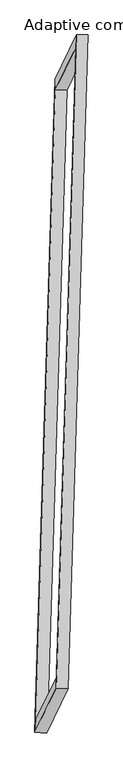
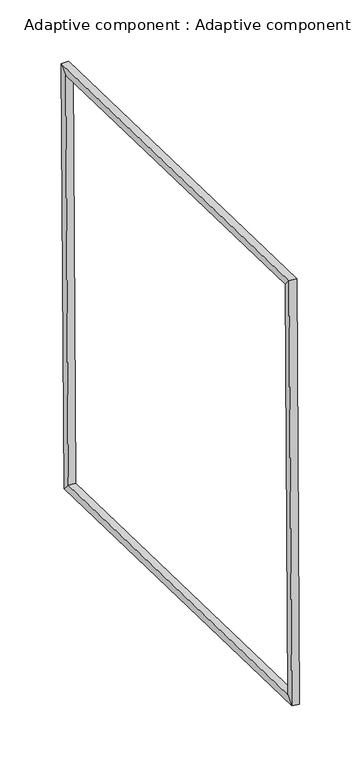
"""IFC4 building model written with IfcOpenShell, lengths in millimetres: proxy geometry, Adaptive component : Adaptive component."""

from ifc_helpers import new_model, si_unit, origin, place, context, project, spatial, faceted_brep, source, transform, mapped, element, save


def adaptive_component_adaptive_component_0c843b08(model_context):
    return source(origin(), model_context, "Body", "Brep", [
        faceted_brep([(93.3015175, 1513.1398614, 3079.6318939), (158.3271165, 1512.9700451, 3079.4089993), (39.2793453, 1267.7769491, -633.5609945), (-25.6282076, 1268.1898956, -629.6563678), (91.0691935, 1444.0024837, 3019.1204679), (-23.7052452, 1207.6108263, -560.5689484), (156.0947925, 1443.8326674, 3018.8975732), (41.2023077, 1207.1978798, -564.473575), (-72.4861012, -2355.6793743, -390.6956056), (-137.2800942, -2351.5847964, -387.0377435), (-131.359767, -2282.5685645, -326.6365646), (-66.565774, -2286.6631424, -330.2944267), (46.5616701, -2110.4862783, 3322.2743882), (-18.3503691, -2106.6348307, 3322.2505182), (-16.5853283, -2046.1769071, 3253.0528516), (48.3267108, -2050.0283548, 3253.0767216)], [[[0, 1, 2, 3]], [[4, 0, 3, 5]], [[6, 4, 5, 7]], [[1, 6, 7, 2]], [[3, 2, 8, 9]], [[5, 3, 9, 10]], [[7, 5, 10, 11]], [[2, 7, 11, 8]], [[9, 8, 12, 13]], [[10, 9, 13, 14]], [[11, 10, 14, 15]], [[8, 11, 15, 12]], [[13, 12, 1, 0]], [[14, 13, 0, 4]], [[15, 14, 4, 6]], [[12, 15, 6, 1]]]),
    ])


if __name__ == "__main__":
    model = new_model("IFC4")
    model_context = context("Model", 3, world=origin())
    ifc_project = project(units=[si_unit("LENGTHUNIT", "METRE", prefix="MILLI")], contexts=[model_context])
    site = spatial("IfcSite", under=ifc_project)
    building = spatial("IfcBuilding", under=site)
    placement = place(None, origin())
    adaptive_component_adaptive_component_shape = adaptive_component_adaptive_component_0c843b08(model_context)
    element("IfcBuildingElementProxy", 1, Name="Adaptive component : Adaptive component", ObjectType="Adaptive component : Adaptive component", at=placement, inside=building, context=model_context, shape_type="MappedRepresentation", body=[
        mapped(adaptive_component_adaptive_component_shape, transform((0.0, 0.0, 0.0), x_axis=(1.0, 0.0, 0.0), y_axis=(0.0, 1.0, 0.0), z_axis=(0.0, 0.0, 1.0))),
    ])
    save(model, "model.ifc")

# Revit data of these elements
# Type "Adaptive component : Adaptive component"
#   r [instance default] = 2063.125 mm
#   2r [instance default] = 4126.251 mm
#   Number [instance default] = 5
#   Default Elevation = 0
# Element 1 (IfcBuildingElementProxy, "Adaptive component : Adaptive component")
#   r = 2506.772 mm
#   2r = 5013.544 mm
#   Number = 21
